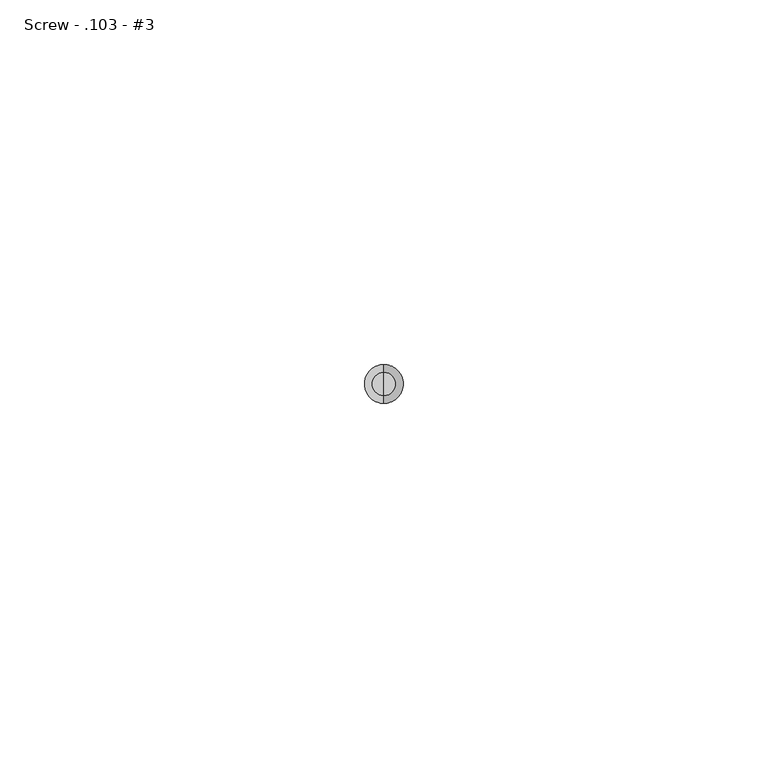
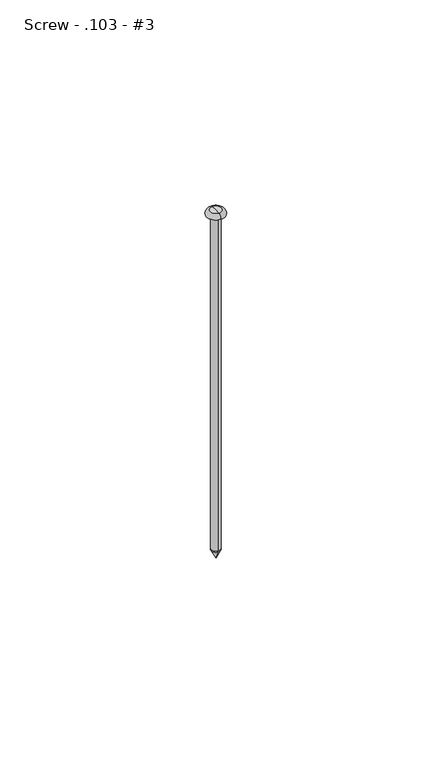
"""IFC4 building model written with IfcOpenShell, lengths in millimetres: fastener geometry, 060523 - W_P_C - Fastenings - Generic : Screw - .103 - #3."""

import ifcopenshell
import ifcopenshell.guid

model = None  # the IFC model being written
_history = None  # IfcOwnerHistory: only IFC2X3 demands one
_inside = {}  # id of a spatial element -> (the spatial element, [elements in it])
_under = {}  # id of a project, library or spatial element -> (it, [spatial elements below it])
_declared = {}  # id of a project -> (the project, [libraries it declares])
_typed = {}  # id of a type object -> (the type object, [elements of that type])
_made_of = {}  # id of a material, layer set ... -> (it, [elements and type objects made of it])


def new_model(schema):
    """Start an empty IFC model of exactly this schema.

    Asked for "IFC4X3", IfcOpenShell would pick the latest addendum, in which some entities
    have other attributes; the version numbers below select the first issue.
    IFC2X3 requires an IfcOwnerHistory on every rooted entity: one is made here for all.
    """
    global model, _history
    if schema == "IFC4X3":
        model = ifcopenshell.file(schema_version=(4, 3, 0, 0))
    else:
        model = ifcopenshell.file(schema=schema)
    _inside.clear()
    _under.clear()
    _declared.clear()
    _typed.clear()
    _made_of.clear()
    _history = None
    if model.schema == "IFC2X3":
        org = make("IfcOrganization", Name="unknown")
        user = make(
            "IfcPersonAndOrganization",
            ThePerson=make("IfcPerson", FamilyName="unknown"),
            TheOrganization=org,
        )
        app = make(
            "IfcApplication",
            ApplicationDeveloper=org,
            Version="unknown",
            ApplicationFullName="unknown",
            ApplicationIdentifier="unknown",
        )
        _history = make(
            "IfcOwnerHistory",
            OwningUser=user,
            OwningApplication=app,
            ChangeAction="ADDED",
            CreationDate=0,
        )
    return model


def make(cls, **values):
    """One entity of the class cls with the attributes given. An attribute that is None is left unset."""
    return model.create_entity(
        cls, **{name: value for name, value in values.items() if value is not None}
    )


def rooted(cls, **values):
    """An entity with a GlobalId (a new one), such as an element, a storey or a relation."""
    return make(cls, GlobalId=ifcopenshell.guid.new(), OwnerHistory=_history, **values)


def si_unit(unit_type, name, prefix=None):
    """IfcSIUnit, for example si_unit("LENGTHUNIT", "METRE", prefix="MILLI")."""
    return make("IfcSIUnit", UnitType=unit_type, Prefix=prefix, Name=name)


def assignment(units):
    """IfcUnitAssignment: the units of a project."""
    return None if units is None else make("IfcUnitAssignment", Units=units)


def point(xyz):
    """IfcCartesianPoint."""
    return None if xyz is None else make("IfcCartesianPoint", Coordinates=xyz)


def direction(xyz):
    """IfcDirection."""
    return None if xyz is None else make("IfcDirection", DirectionRatios=xyz)


def frame(location, z_axis=None, x_axis=None):
    """IfcAxis2Placement3D, a coordinate frame: its origin and axes. An axis left out is left unset."""
    return make(
        "IfcAxis2Placement3D",
        Location=point(location),
        Axis=direction(z_axis),
        RefDirection=direction(x_axis),
    )


def frame_2d(location, x_axis=None):
    """IfcAxis2Placement2D, a coordinate frame in the plane: its origin and x axis."""
    return make(
        "IfcAxis2Placement2D", Location=point(location), RefDirection=direction(x_axis)
    )


def origin():
    """The frame at (0, 0, 0) with its axes left unset."""
    return frame((0.0, 0.0, 0.0))


def origin_2d():
    """The frame at (0, 0) in the plane with its x axis left unset."""
    return frame_2d((0.0, 0.0))


def place(relative_to, where):
    """IfcLocalPlacement: puts the frame where relative to a parent placement (None: the world)."""
    return make(
        "IfcLocalPlacement", PlacementRelTo=relative_to, RelativePlacement=where
    )


def context(
    kind, dimensions, precision=None, world=None, true_north=None, identifier=None
):
    """IfcGeometricRepresentationContext, for example the 3D "Model" context."""
    return make(
        "IfcGeometricRepresentationContext",
        ContextIdentifier=identifier,
        ContextType=kind,
        CoordinateSpaceDimension=dimensions,
        Precision=precision,
        WorldCoordinateSystem=world,
        TrueNorth=true_north,
    )


def project(units=None, contexts=None):
    """IfcProject with its units and contexts."""
    return rooted(
        "IfcProject",
        Name="project",
        RepresentationContexts=contexts,
        UnitsInContext=assignment(units),
    )


def spatial(cls, under=None, at=None, **own):
    """A site, building, storey or space (cls), placed at a placement, below another one or the project."""
    s = rooted(cls, ObjectPlacement=at, **own)
    if under is not None:
        _under.setdefault(under.id(), (under, []))[1].append(s)
    return s


def polyline(points):
    """IfcPolyline through the points."""
    return make("IfcPolyline", Points=[point(p) for p in points])


def circle_curve(where, radius):
    """IfcCircle in the frame where."""
    return make("IfcCircle", Position=where, Radius=radius)


def ellipse_curve(where, semi_axis1, semi_axis2):
    """IfcEllipse in the frame where."""
    return make(
        "IfcEllipse", Position=where, SemiAxis1=semi_axis1, SemiAxis2=semi_axis2
    )


def trimmed(basis, trim1, trim2, sense, master):
    """IfcTrimmedCurve: the piece of a basis curve between two trims."""
    return make(
        "IfcTrimmedCurve",
        BasisCurve=basis,
        Trim1=trim1,
        Trim2=trim2,
        SenseAgreement=sense,
        MasterRepresentation=master,
    )


def segment(curve, same_sense, transition):
    """IfcCompositeCurveSegment."""
    return make(
        "IfcCompositeCurveSegment",
        Transition=transition,
        SameSense=same_sense,
        ParentCurve=curve,
    )


def composite_curve(segments, self_intersect=None):
    """IfcCompositeCurve: segments joined end to end."""
    return make("IfcCompositeCurve", Segments=segments, SelfIntersect=self_intersect)


def outline(outer, holes=None, kind="AREA"):
    """IfcArbitraryClosedProfileDef: a profile drawn as a closed curve; with holes, ...WithVoids."""
    if holes is None:
        return make("IfcArbitraryClosedProfileDef", ProfileType=kind, OuterCurve=outer)
    return make(
        "IfcArbitraryProfileDefWithVoids",
        ProfileType=kind,
        OuterCurve=outer,
        InnerCurves=holes,
    )


def extrude(swept, where, along, depth):
    """IfcExtrudedAreaSolid: the profile swept, set in the frame where, extruded along a direction by depth."""
    return make(
        "IfcExtrudedAreaSolid",
        SweptArea=swept,
        Position=where,
        ExtrudedDirection=direction(along),
        Depth=depth,
    )


def shape(context_of_items, identifier, shape_type, items):
    """IfcShapeRepresentation: the items that make up one representation, for example the "Body"."""
    return make(
        "IfcShapeRepresentation",
        ContextOfItems=context_of_items,
        RepresentationIdentifier=identifier,
        RepresentationType=shape_type,
        Items=items,
    )


def source(mapping_origin, context_of_items, identifier, shape_type, items):
    """IfcRepresentationMap: a shape defined once, which mapped items show again and again."""
    return make(
        "IfcRepresentationMap",
        MappingOrigin=mapping_origin,
        MappedRepresentation=shape(context_of_items, identifier, shape_type, items),
    )


def transform(
    local_origin,
    x_axis=None,
    y_axis=None,
    z_axis=None,
    scale=None,
    scale2=None,
    scale3=None,
    uniform=True,
):
    """IfcCartesianTransformationOperator3D, or its non-uniform kind. x_axis, y_axis, z_axis: its Axis1, 2, 3."""
    if uniform:
        return make(
            "IfcCartesianTransformationOperator3D",
            Axis1=direction(x_axis),
            Axis2=direction(y_axis),
            LocalOrigin=point(local_origin),
            Scale=scale,
            Axis3=direction(z_axis),
        )
    return make(
        "IfcCartesianTransformationOperator3DnonUniform",
        Axis1=direction(x_axis),
        Axis2=direction(y_axis),
        LocalOrigin=point(local_origin),
        Scale=scale,
        Axis3=direction(z_axis),
        Scale2=scale2,
        Scale3=scale3,
    )


def mapped(mapping_source, mapping_target):
    """IfcMappedItem: shows the shape of a source again, moved by a transform."""
    return make(
        "IfcMappedItem", MappingSource=mapping_source, MappingTarget=mapping_target
    )


def made_of(thing, what):
    """Note that an element or type object is made of a material, layer set ...; save() writes the relation."""
    if what is not None:
        _made_of.setdefault(what.id(), (what, []))[1].append(thing)
    return thing


def element(
    cls,
    number,
    at=None,
    inside=None,
    cuts=None,
    type_object=None,
    material=None,
    context=None,
    identifier="Body",
    shape_type=None,
    held_by="IfcProductDefinitionShape",
    body=None,
    shapes=None,
    **own,
):
    """One element of the class cls, such as IfcWall. Its Tag is "e" and its number.

    at: its placement. inside: the storey or other place that contains it. cuts: it is an
    opening in that element (IfcRelVoidsElement). A single representation is given by context,
    identifier, shape_type and body (its items); several are given by shapes. held_by: the class
    of the entity that holds the representations. save() writes the other relations.
    """
    e = rooted(cls, Tag="e%d" % number, ObjectPlacement=at, **own)
    if body is not None:
        shapes = [shape(context, identifier, shape_type, body)]
    if shapes is not None:
        e.Representation = make(held_by, Representations=shapes)
    if inside is not None:
        _inside.setdefault(inside.id(), (inside, []))[1].append(e)
    if cuts is not None:
        rooted(
            "IfcRelVoidsElement", RelatingBuildingElement=cuts, RelatedOpeningElement=e
        )
    if type_object is not None:
        _typed.setdefault(type_object.id(), (type_object, []))[1].append(e)
    return made_of(e, material)


def aggregate(whole, parts):
    """IfcRelAggregates: a whole, such as a stair, and the parts it consists of."""
    return rooted("IfcRelAggregates", RelatingObject=whole, RelatedObjects=parts)


def save(model, path):
    """Write the relations noted so far, then the file.

    IfcRelAggregates (storeys below a building ...), IfcRelContainedInSpatialStructure (elements
    in a storey), IfcRelDefinesByType, IfcRelAssociatesMaterial and IfcRelDeclares: one each for
    every whole, place, type object, material and project.
    """
    for whole, parts in _under.values():
        aggregate(whole, parts)
    for where, things in _inside.values():
        rooted(
            "IfcRelContainedInSpatialStructure",
            RelatedElements=things,
            RelatingStructure=where,
        )
    for kind, things in _typed.values():
        rooted("IfcRelDefinesByType", RelatedObjects=things, RelatingType=kind)
    for what, things in _made_of.values():
        rooted("IfcRelAssociatesMaterial", RelatedObjects=things, RelatingMaterial=what)
    for by, libraries in _declared.values():
        rooted("IfcRelDeclares", RelatingContext=by, RelatedDefinitions=libraries)
    model.write(path)


def plane_surface(at):
    """IfcPlane: the flat surface through the origin of the frame at, square to its z axis."""
    return make("IfcPlane", Position=at)


def revolved_surface(curve, axis_point, axis_direction):
    """IfcSurfaceOfRevolution: the curve turned about the line through axis_point along axis_direction."""
    return make(
        "IfcSurfaceOfRevolution",
        SweptCurve=make("IfcArbitraryOpenProfileDef", ProfileType="CURVE", Curve=curve),
        AxisPosition=make("IfcAxis1Placement", Location=point(axis_point), Axis=direction(axis_direction)),
    )


def advanced_brep(points, edges, surfaces, faces):
    """IfcAdvancedBrep: a solid bounded by faces that lie on surfaces and meet in shared edges.

    An edge is (start, end): straight between two places in points (the first is 0);
    or (start, end, curve); or (start, end, curve, False) where it runs against its curve.
    A face is (place in surfaces, loops), or (place, loops, False) where it looks against
    its surface's normal. A loop lists edges by number (the first is 1), with a minus sign
    where the edge is run from its end to its start. The first loop is the outer one.
    """
    corners = [point(p) for p in points]
    vertices = [make("IfcVertexPoint", VertexGeometry=c) for c in corners]
    made = []
    for start, end, *more in edges:
        made.append(
            make(
                "IfcEdgeCurve",
                EdgeStart=vertices[start],
                EdgeEnd=vertices[end],
                EdgeGeometry=more[0] if more else make("IfcPolyline", Points=[corners[start], corners[end]]),
                SameSense=more[1] if len(more) > 1 else True,
            )
        )
    hull = []
    for where, loops, *sense in faces:
        bounds = []
        for j, loop in enumerate(loops):
            ring = [make("IfcOrientedEdge", EdgeElement=made[abs(k) - 1], Orientation=k > 0) for k in loop]
            bounds.append(
                make(
                    "IfcFaceOuterBound" if j == 0 else "IfcFaceBound",
                    Bound=make("IfcEdgeLoop", EdgeList=ring),
                    Orientation=True,
                )
            )
        hull.append(make("IfcAdvancedFace", Bounds=bounds, FaceSurface=surfaces[where], SameSense=sense[0] if sense else True))
    return make("IfcAdvancedBrep", Outer=make("IfcClosedShell", CfsFaces=hull))


def screw_103_3_e6721dde(model_context):
    return source(origin(), model_context, "Body", "SolidModel", [
        advanced_brep(
        [(0.0, -1.3081, -101.6), (0.0, 1.3081, -101.6), (0.0, 0.0, -101.6), (0.0, 0.0, -104.2162)],
        [
            (0, 1, circle_curve(frame((0.0, 0.0, -101.6), z_axis=(0.0, 0.0, 1.0), x_axis=(0.0, 1.0, 0.0)), 1.3081)),
            (1, 2),
            (2, 0),
            (1, 0, circle_curve(frame((0.0, 0.0, -101.6), z_axis=(0.0, 0.0, 1.0), x_axis=(0.0, 1.0, 0.0)), 1.3081)),
            (3, 1),
            (0, 3),
        ],
        [
            plane_surface(frame((0.0, 0.0, -101.6), z_axis=(0.0, 0.0, 1.0), x_axis=(0.0, 1.0, 0.0))),
            revolved_surface(polyline([(0.0, 1.3081, -101.6), (0.0, 0.0, -104.2162)]), (0.0, 0.0, -103.0840259), (0.0, 0.0, -1.0)),
        ],
        [
            (0, [[1, 2, 3]]),
            (0, [[4, -3, -2]]),
            (1, [[5, -1, 6]]),
            (1, [[-6, -4, -5]]),
        ],
    ),
        advanced_brep(
        [(0.0, 2.6162, 0.0), (0.0, -2.6162, 0.0), (0.0, 0.0, 0.0), (0.0, 0.0, 1.3081), (0.0, -1.5875, 1.3081), (0.0, 1.5875, 1.3081)],
        [
            (0, 1, circle_curve(frame((0.0, 0.0, 0.0), z_axis=(0.0, 0.0, -1.0), x_axis=(0.0, -1.0, 0.0)), 2.6162)),
            (1, 2),
            (2, 0),
            (1, 0, circle_curve(frame((0.0, 0.0, 0.0), z_axis=(0.0, 0.0, -1.0), x_axis=(0.0, -1.0, 0.0)), 2.6162)),
            (3, 4),
            (4, 5, circle_curve(frame((0.0, 0.0, 1.3081), z_axis=(0.0, 0.0, 1.0), x_axis=(0.0, -1.0, 0.0)), 1.5875)),
            (5, 3),
            (5, 4, circle_curve(frame((0.0, 0.0, 1.3081), z_axis=(0.0, 0.0, 1.0), x_axis=(0.0, -1.0, 0.0)), 1.5875)),
            (4, 1, circle_curve(frame((0.0, -1.5875, 0.2495612), z_axis=(1.0, 0.0, 0.0), x_axis=(0.0, -1.0, 0.0)), 1.0585388)),
            (0, 5, circle_curve(frame((0.0, 1.5875, 0.2495612), z_axis=(1.0, 0.0, 0.0), x_axis=(0.0, 1.0, 0.0)), 1.0585388)),
        ],
        [
            plane_surface(frame((0.0, 0.0, 0.0), z_axis=(0.0, 0.0, -1.0), x_axis=(0.0, -1.0, 0.0))),
            plane_surface(frame((0.0, 0.0, 1.3081), z_axis=(0.0, 0.0, 1.0), x_axis=(0.0, -1.0, 0.0))),
            revolved_surface(trimmed(ellipse_curve(frame((0.0, -1.5875, 0.2495612), z_axis=(-1.0, 0.0, 0.0), x_axis=(0.0, -1.0, 0.0)), 1.0585388, 1.0585388), [point((0.0, -2.6162, 0.0))], [point((0.0, -1.5875, 1.3081))], True, "CARTESIAN"), (0.0, 0.0, 1.4840259), (0.0, 0.0, 1.0)),
        ],
        [
            (0, [[1, 2, 3]]),
            (0, [[4, -3, -2]]),
            (1, [[5, 6, 7]]),
            (1, [[-7, 8, -5]]),
            (2, [[-6, 9, -1, 10]]),
            (2, [[-8, -10, -4, -9]]),
        ],
    ),
        extrude(outline(composite_curve([segment(trimmed(circle_curve(origin_2d(), 1.3081), [point((0.0, -1.3081))], [point((0.0, 1.3081))], False, "CARTESIAN"), True, "CONTINUOUS"), segment(trimmed(circle_curve(origin_2d(), 1.3081), [point((0.0, 1.3081))], [point((0.0, -1.3081))], False, "CARTESIAN"), True, "CONTINUOUS")], self_intersect=False)), frame((0.0, 0.0, -101.6), z_axis=(0.0, 0.0, 1.0), x_axis=(1.0, 0.0, 0.0)), (0.0, 0.0, 1.0), 101.6),
    ])


if __name__ == "__main__":
    model = new_model("IFC4")
    model_context = context("Model", 3, world=origin())
    ifc_project = project(units=[si_unit("LENGTHUNIT", "METRE", prefix="MILLI")], contexts=[model_context])
    site = spatial("IfcSite", under=ifc_project)
    building = spatial("IfcBuilding", under=site)
    placement = place(None, origin())
    screw_103_3_shape = screw_103_3_e6721dde(model_context)
    element("IfcFastener", 1, ObjectType="060523 - W_P_C - Fastenings - Generic : Screw - .103 - #3", at=placement, inside=building, context=model_context, shape_type="MappedRepresentation", body=[
        mapped(screw_103_3_shape, transform((0.0, 0.0, 0.0), x_axis=(1.0, 0.0, 0.0), y_axis=(0.0, 1.0, 0.0), z_axis=(0.0, 0.0, 1.0))),
    ])
    save(model, "model.ifc")

# Revit data of these elements
# Type "060523 - W_P_C - Fastenings - Generic : Screw - .103 - #3"
#   Washer_Thickness = 0' - 0.00333"
#   Washer Radius = 0' - 0.0615"
#   Washer Offset - Head = 0' - 0"
#   Washer Offset = 0' - 0"
#   Thickness_of_Substrate [instance default] = 0' - 1"
#   Side = 0' - 0 37/64"
#   Radius = 0' - 0.0515"
#   Length [instance default] = 0' - 4"
#   Head Size = 0' - 1"
#   Head Radius = 0' - 0 1/2"
#   Head Height = 0' - 0.01"
#   Double Diameter = 0' - 0.206"
#   Diameter = 0' - 0.103"
#   Default Elevation = 4' - 0"
#   Washer_Nut_Visibility = no
#   Washer_Head_Visibility = no
#   Round_Head_Visibility = yes
#   Point Visibility = yes
#   Nut_Visibility = no
#   Hex_Head_Visiblilty = no
#   Washer Material = none
#   Bolt Material (Size) = AT SILL - FASTENER AT 24" O.C.
# Element 1 (IfcFastener, "060523 - W_P_C - Fastenings - Generic : Screw - .103 - #3")
#   Materials on its faces: "AT SILL - FASTENER AT 24\" O.C."
# Materials
#   "AT SILL - FASTENER AT 24\" O.C.": class "Generic", colour RGB 120 120 120, transparency 0, Cost = 0
